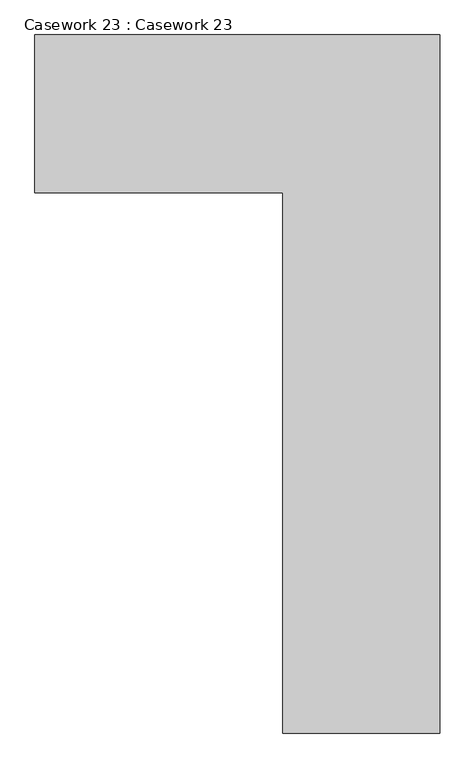
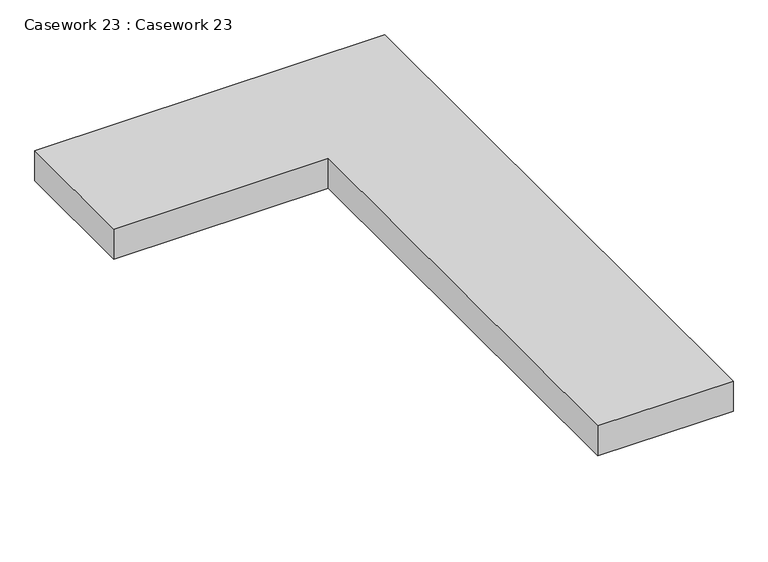
"""IFC4 building model written with IfcOpenShell, lengths in millimetres: furniture geometry, Casework 23 : Casework 23."""

from ifc_helpers import new_model, si_unit, frame, origin, place, context, project, spatial, polyline, outline, extrude, source, transform, mapped, element, save


def casework_23_casework_23_04205953(model_context):
    return source(origin(), model_context, "Body", "SweptSolid", [
        extrude(outline(polyline([(-34032.6785979, 281388.6385405), (-35332.055403, 281388.6385405), (-35332.055403, 285870.0613827), (-37389.4539888, 285870.0613827), (-37389.4539888, 287179.7737113), (-34032.6785979, 287179.7737113), (-34032.6785979, 281388.6385405)])), frame((0.0, 0.0, 3048.0), z_axis=(0.0, 0.0, 1.0), x_axis=(1.0, 0.0, 0.0)), (0.0, 0.0, 1.0), 305.2489812),
    ])


if __name__ == "__main__":
    model = new_model("IFC4")
    model_context = context("Model", 3, world=origin())
    ifc_project = project(units=[si_unit("LENGTHUNIT", "METRE", prefix="MILLI")], contexts=[model_context])
    site = spatial("IfcSite", under=ifc_project)
    building = spatial("IfcBuilding", under=site)
    placement = place(None, origin())
    casework_23_casework_23_shape = casework_23_casework_23_04205953(model_context)
    element("IfcFurniture", 1, ObjectType="Casework 23 : Casework 23", at=placement, inside=building, context=model_context, shape_type="MappedRepresentation", body=[
        mapped(casework_23_casework_23_shape, transform((0.0, 0.0, 0.0), x_axis=(1.0, 0.0, 0.0), y_axis=(0.0, 1.0, 0.0), z_axis=(0.0, 0.0, 1.0))),
    ])
    save(model, "model.ifc")

# Revit data of these elements
# Element 1 (IfcFurniture, "Casework 23 : Casework 23")
#   Materials on its faces: "Dark metal"
# Materials
#   "Dark metal": class "Generic", colour RGB 44 29 29, transparency 0, Cost = 0
